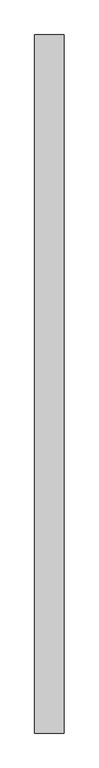
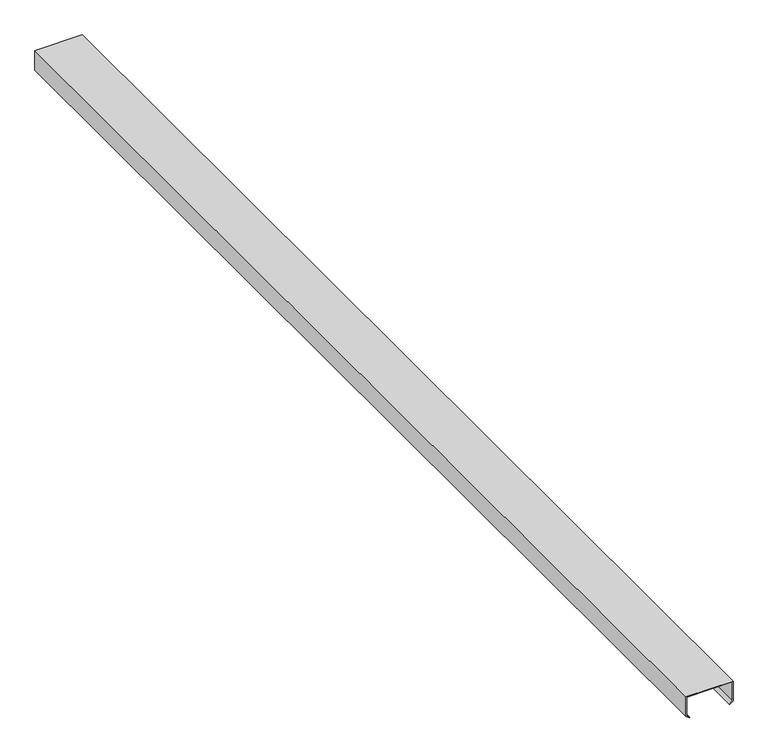
"""IFC4 building model written with IfcOpenShell, lengths in millimetres: proxy geometry, Generic Models 7:Generic Models 1:1:Generic Models 1:1 : Generic Models 7:Generic Models 1:337419:18 : Generic Models 7:Generic Models 1:1:Generic Models 1:1 : Generic Models 7:Generic Models 1:337419:306201."""

import ifcopenshell
import ifcopenshell.guid

model = None  # the IFC model being written
_history = None  # IfcOwnerHistory: only IFC2X3 demands one
_inside = {}  # id of a spatial element -> (the spatial element, [elements in it])
_under = {}  # id of a project, library or spatial element -> (it, [spatial elements below it])
_declared = {}  # id of a project -> (the project, [libraries it declares])
_typed = {}  # id of a type object -> (the type object, [elements of that type])
_made_of = {}  # id of a material, layer set ... -> (it, [elements and type objects made of it])


def new_model(schema):
    """Start an empty IFC model of exactly this schema.

    Asked for "IFC4X3", IfcOpenShell would pick the latest addendum, in which some entities
    have other attributes; the version numbers below select the first issue.
    IFC2X3 requires an IfcOwnerHistory on every rooted entity: one is made here for all.
    """
    global model, _history
    if schema == "IFC4X3":
        model = ifcopenshell.file(schema_version=(4, 3, 0, 0))
    else:
        model = ifcopenshell.file(schema=schema)
    _inside.clear()
    _under.clear()
    _declared.clear()
    _typed.clear()
    _made_of.clear()
    _history = None
    if model.schema == "IFC2X3":
        org = make("IfcOrganization", Name="unknown")
        user = make(
            "IfcPersonAndOrganization",
            ThePerson=make("IfcPerson", FamilyName="unknown"),
            TheOrganization=org,
        )
        app = make(
            "IfcApplication",
            ApplicationDeveloper=org,
            Version="unknown",
            ApplicationFullName="unknown",
            ApplicationIdentifier="unknown",
        )
        _history = make(
            "IfcOwnerHistory",
            OwningUser=user,
            OwningApplication=app,
            ChangeAction="ADDED",
            CreationDate=0,
        )
    return model


def make(cls, **values):
    """One entity of the class cls with the attributes given. An attribute that is None is left unset."""
    return model.create_entity(
        cls, **{name: value for name, value in values.items() if value is not None}
    )


def rooted(cls, **values):
    """An entity with a GlobalId (a new one), such as an element, a storey or a relation."""
    return make(cls, GlobalId=ifcopenshell.guid.new(), OwnerHistory=_history, **values)


def si_unit(unit_type, name, prefix=None):
    """IfcSIUnit, for example si_unit("LENGTHUNIT", "METRE", prefix="MILLI")."""
    return make("IfcSIUnit", UnitType=unit_type, Prefix=prefix, Name=name)


def assignment(units):
    """IfcUnitAssignment: the units of a project."""
    return None if units is None else make("IfcUnitAssignment", Units=units)


def point(xyz):
    """IfcCartesianPoint."""
    return None if xyz is None else make("IfcCartesianPoint", Coordinates=xyz)


def direction(xyz):
    """IfcDirection."""
    return None if xyz is None else make("IfcDirection", DirectionRatios=xyz)


def frame(location, z_axis=None, x_axis=None):
    """IfcAxis2Placement3D, a coordinate frame: its origin and axes. An axis left out is left unset."""
    return make(
        "IfcAxis2Placement3D",
        Location=point(location),
        Axis=direction(z_axis),
        RefDirection=direction(x_axis),
    )


def origin():
    """The frame at (0, 0, 0) with its axes left unset."""
    return frame((0.0, 0.0, 0.0))


def place(relative_to, where):
    """IfcLocalPlacement: puts the frame where relative to a parent placement (None: the world)."""
    return make(
        "IfcLocalPlacement", PlacementRelTo=relative_to, RelativePlacement=where
    )


def context(
    kind, dimensions, precision=None, world=None, true_north=None, identifier=None
):
    """IfcGeometricRepresentationContext, for example the 3D "Model" context."""
    return make(
        "IfcGeometricRepresentationContext",
        ContextIdentifier=identifier,
        ContextType=kind,
        CoordinateSpaceDimension=dimensions,
        Precision=precision,
        WorldCoordinateSystem=world,
        TrueNorth=true_north,
    )


def project(units=None, contexts=None):
    """IfcProject with its units and contexts."""
    return rooted(
        "IfcProject",
        Name="project",
        RepresentationContexts=contexts,
        UnitsInContext=assignment(units),
    )


def spatial(cls, under=None, at=None, **own):
    """A site, building, storey or space (cls), placed at a placement, below another one or the project."""
    s = rooted(cls, ObjectPlacement=at, **own)
    if under is not None:
        _under.setdefault(under.id(), (under, []))[1].append(s)
    return s


def polyline(points):
    """IfcPolyline through the points."""
    return make("IfcPolyline", Points=[point(p) for p in points])


def outline(outer, holes=None, kind="AREA"):
    """IfcArbitraryClosedProfileDef: a profile drawn as a closed curve; with holes, ...WithVoids."""
    if holes is None:
        return make("IfcArbitraryClosedProfileDef", ProfileType=kind, OuterCurve=outer)
    return make(
        "IfcArbitraryProfileDefWithVoids",
        ProfileType=kind,
        OuterCurve=outer,
        InnerCurves=holes,
    )


def extrude(swept, where, along, depth):
    """IfcExtrudedAreaSolid: the profile swept, set in the frame where, extruded along a direction by depth."""
    return make(
        "IfcExtrudedAreaSolid",
        SweptArea=swept,
        Position=where,
        ExtrudedDirection=direction(along),
        Depth=depth,
    )


def shape(context_of_items, identifier, shape_type, items):
    """IfcShapeRepresentation: the items that make up one representation, for example the "Body"."""
    return make(
        "IfcShapeRepresentation",
        ContextOfItems=context_of_items,
        RepresentationIdentifier=identifier,
        RepresentationType=shape_type,
        Items=items,
    )


def source(mapping_origin, context_of_items, identifier, shape_type, items):
    """IfcRepresentationMap: a shape defined once, which mapped items show again and again."""
    return make(
        "IfcRepresentationMap",
        MappingOrigin=mapping_origin,
        MappedRepresentation=shape(context_of_items, identifier, shape_type, items),
    )


def transform(
    local_origin,
    x_axis=None,
    y_axis=None,
    z_axis=None,
    scale=None,
    scale2=None,
    scale3=None,
    uniform=True,
):
    """IfcCartesianTransformationOperator3D, or its non-uniform kind. x_axis, y_axis, z_axis: its Axis1, 2, 3."""
    if uniform:
        return make(
            "IfcCartesianTransformationOperator3D",
            Axis1=direction(x_axis),
            Axis2=direction(y_axis),
            LocalOrigin=point(local_origin),
            Scale=scale,
            Axis3=direction(z_axis),
        )
    return make(
        "IfcCartesianTransformationOperator3DnonUniform",
        Axis1=direction(x_axis),
        Axis2=direction(y_axis),
        LocalOrigin=point(local_origin),
        Scale=scale,
        Axis3=direction(z_axis),
        Scale2=scale2,
        Scale3=scale3,
    )


def mapped(mapping_source, mapping_target):
    """IfcMappedItem: shows the shape of a source again, moved by a transform."""
    return make(
        "IfcMappedItem", MappingSource=mapping_source, MappingTarget=mapping_target
    )


def made_of(thing, what):
    """Note that an element or type object is made of a material, layer set ...; save() writes the relation."""
    if what is not None:
        _made_of.setdefault(what.id(), (what, []))[1].append(thing)
    return thing


def element(
    cls,
    number,
    at=None,
    inside=None,
    cuts=None,
    type_object=None,
    material=None,
    context=None,
    identifier="Body",
    shape_type=None,
    held_by="IfcProductDefinitionShape",
    body=None,
    shapes=None,
    **own,
):
    """One element of the class cls, such as IfcWall. Its Tag is "e" and its number.

    at: its placement. inside: the storey or other place that contains it. cuts: it is an
    opening in that element (IfcRelVoidsElement). A single representation is given by context,
    identifier, shape_type and body (its items); several are given by shapes. held_by: the class
    of the entity that holds the representations. save() writes the other relations.
    """
    e = rooted(cls, Tag="e%d" % number, ObjectPlacement=at, **own)
    if body is not None:
        shapes = [shape(context, identifier, shape_type, body)]
    if shapes is not None:
        e.Representation = make(held_by, Representations=shapes)
    if inside is not None:
        _inside.setdefault(inside.id(), (inside, []))[1].append(e)
    if cuts is not None:
        rooted(
            "IfcRelVoidsElement", RelatingBuildingElement=cuts, RelatedOpeningElement=e
        )
    if type_object is not None:
        _typed.setdefault(type_object.id(), (type_object, []))[1].append(e)
    return made_of(e, material)


def aggregate(whole, parts):
    """IfcRelAggregates: a whole, such as a stair, and the parts it consists of."""
    return rooted("IfcRelAggregates", RelatingObject=whole, RelatedObjects=parts)


def save(model, path):
    """Write the relations noted so far, then the file.

    IfcRelAggregates (storeys below a building ...), IfcRelContainedInSpatialStructure (elements
    in a storey), IfcRelDefinesByType, IfcRelAssociatesMaterial and IfcRelDeclares: one each for
    every whole, place, type object, material and project.
    """
    for whole, parts in _under.values():
        aggregate(whole, parts)
    for where, things in _inside.values():
        rooted(
            "IfcRelContainedInSpatialStructure",
            RelatedElements=things,
            RelatingStructure=where,
        )
    for kind, things in _typed.values():
        rooted("IfcRelDefinesByType", RelatedObjects=things, RelatingType=kind)
    for what, things in _made_of.values():
        rooted("IfcRelAssociatesMaterial", RelatedObjects=things, RelatingMaterial=what)
    for by, libraries in _declared.values():
        rooted("IfcRelDeclares", RelatingContext=by, RelatedDefinitions=libraries)
    model.write(path)


def generic_models_6bc2a326(model_context):
    return source(origin(), model_context, "Body", "SweptSolid", [
        extrude(outline(polyline([(4985.940625, 579307.711724), (4985.940625, 579104.511724), (4897.040625, 579104.511724), (4884.7955211, 579119.1048707), (4886.9236883, 579120.890615), (4898.336086, 579107.289849), (4983.1625, 579107.289849), (4983.1625, 579304.933599), (4898.336086, 579304.933599), (4886.9236883, 579291.3328331), (4884.7955211, 579293.1185774), (4897.040625, 579307.711724), (4985.940625, 579307.711724)])), frame((0.0, -578797.4913841, 0.0), z_axis=(0.0, 1.0, 0.0), x_axis=(0.0, 0.0, 1.0)), (0.0, 0.0, 1.0), 4854.575),
    ])


if __name__ == "__main__":
    model = new_model("IFC4")
    model_context = context("Model", 3, world=origin())
    ifc_project = project(units=[si_unit("LENGTHUNIT", "METRE", prefix="MILLI")], contexts=[model_context])
    site = spatial("IfcSite", under=ifc_project)
    building = spatial("IfcBuilding", under=site)
    placement = place(None, origin())
    generic_models_shape = generic_models_6bc2a326(model_context)
    element("IfcBuildingElementProxy", 1, Name="Generic Models 7:Generic Models 1:1:Generic Models 1:1 : Generic Models 7:Generic Models 1:337419:18 : Generic Models 7:Generic Models 1:1:Generic Models 1:1 : Generic Models 7:Generic Models 1:337419:306201", ObjectType="Generic Models 7:Generic Models 1:1:Generic Models 1:1 : Generic Models 7:Generic Models 1:337419:18 : Generic Models 7:Generic Models 1:1:Generic Models 1:1 : Generic Models 7:Generic Models 1:337419:306201", at=placement, inside=building, context=model_context, shape_type="MappedRepresentation", body=[
        mapped(generic_models_shape, transform((0.0, 0.0, 0.0), x_axis=(1.0, 0.0, 0.0), y_axis=(0.0, 1.0, 0.0), z_axis=(0.0, 0.0, 1.0))),
    ])
    save(model, "model.ifc")

# Revit data of these elements
# Type "Generic Models 7:Generic Models 1:1:Generic Models 1:1 : Generic Models 7:Generic Models 1:337419:18 : Generic Models 7:Generic Models 1:1:Generic Models 1:1 : Generic Models 7:Generic Models 1:337419:306201"
#   NameOverride = "Generic Models 7:Generic Models 1:1:Generic Models 1:1 : Generic Models 7:Generic Models 1:337419:306201"
#   ObjectTypeOverride = "Generic Models 1:1 : Generic Models 7:Generic Models 1:337419"
#   Reference = "Generic Models 1"
#   Tag = "306201"
# Element 1 (IfcBuildingElementProxy, "Generic Models 7:Generic Models 1:1:Generic Models 1:1 : Generic Models 7:Generic Models 1:337419:18 : Generic Models 7:Generic Models 1:1:Generic Models 1:1 : Generic Models 7:Generic Models 1:337419:306201")
#   Materials on its faces: "'ZEE' SECTION (8.0x3.5Z - SEE STRUCT. DWGS)"
# Materials
#   "'ZEE' SECTION (8.0x3.5Z - SEE STRUCT. DWGS)": class "Unassigned", colour RGB 210 209 208, transparency 0, Keynote = "M05121300.02", Cost = 0
